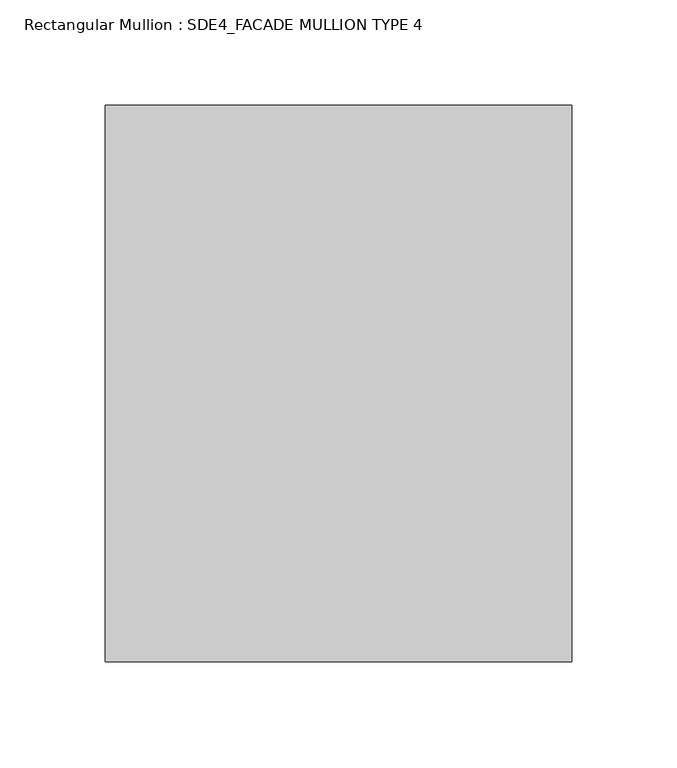
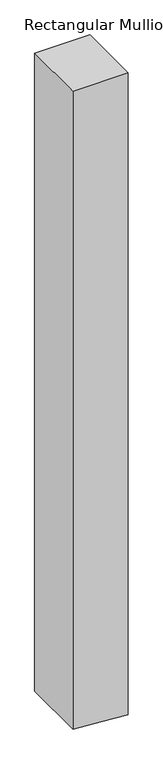
"""IFC4 building model written with IfcOpenShell, lengths in millimetres: member geometry, Rectangular Mullion : SDE4_FACADE MULLION TYPE 4."""

from ifc_helpers import new_model, si_unit, frame, origin, place, context, project, spatial, polyline, outline, extrude, source, transform, mapped, element, save


def rectangular_mullion_sde4_facade_mullion_type_4_7bc08063(model_context):
    return source(origin(), model_context, "Body", "SweptSolid", [
        extrude(outline(polyline([(0.0, 111.0), (0.0, -111.0), (-2708.9029211, -111.0), (-2717.6438427, 3.056508), (-2725.9162826, 111.0), (0.0, 111.0)])), frame((0.0, -132.5, 0.0), z_axis=(0.0, 1.0, 0.0), x_axis=(0.0, 0.0, 1.0)), (0.0, 0.0, 1.0), 265.0),
    ])


if __name__ == "__main__":
    model = new_model("IFC4")
    model_context = context("Model", 3, world=origin())
    ifc_project = project(units=[si_unit("LENGTHUNIT", "METRE", prefix="MILLI")], contexts=[model_context])
    site = spatial("IfcSite", under=ifc_project)
    building = spatial("IfcBuilding", under=site)
    placement = place(None, origin())
    rectangular_mullion_sde4_facade_mullion_type_4_shape = rectangular_mullion_sde4_facade_mullion_type_4_7bc08063(model_context)
    element("IfcMember", 1, ObjectType="Rectangular Mullion : SDE4_FACADE MULLION TYPE 4", at=placement, inside=building, context=model_context, shape_type="MappedRepresentation", body=[
        mapped(rectangular_mullion_sde4_facade_mullion_type_4_shape, transform((0.0, 0.0, 0.0), x_axis=(1.0, 0.0, 0.0), y_axis=(0.0, 1.0, 0.0), z_axis=(0.0, 0.0, 1.0))),
    ])
    save(model, "model.ifc")

# Revit data of these elements
# Type "Rectangular Mullion : SDE4_FACADE MULLION TYPE 4"
#   built-in parameter 1007322 = 0.869423 (stored number, unit not read)
#   built-in parameter 1007321 = 0.364173 (stored number, unit not read)
#   built-in parameter 1007320 = 0.364173 (stored number, unit not read)
